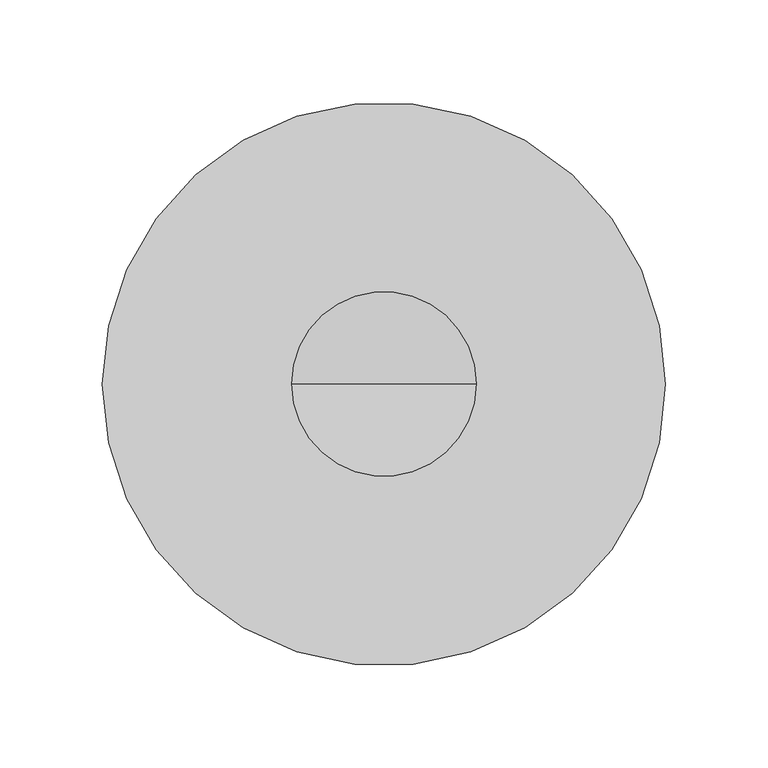
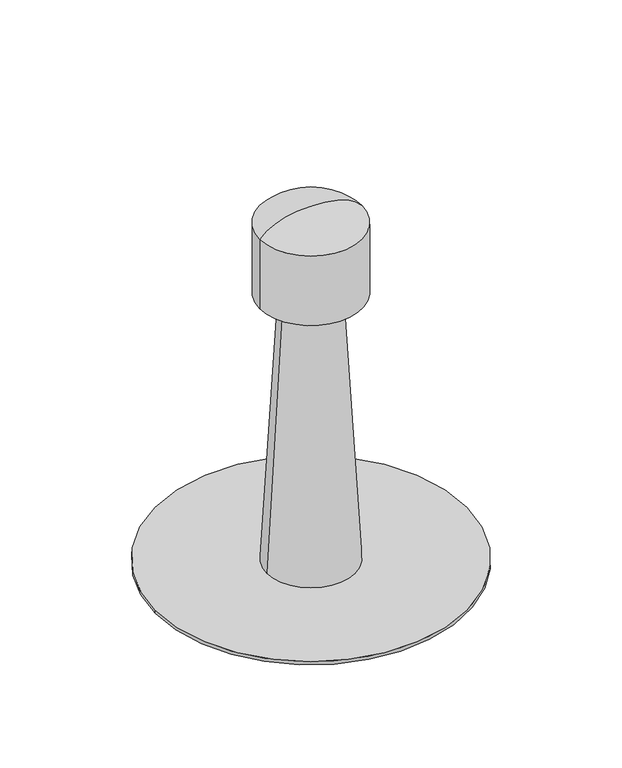
"""IFC4 building model written with IfcOpenShell, lengths in millimetres: proxy geometry, TN_ПВХ Кровельный аэратор : ПВХ аэратор кровельный 78х332 ТехноНИКОЛЬ."""

import ifcopenshell
import ifcopenshell.guid

model = None  # the IFC model being written
_history = None  # IfcOwnerHistory: only IFC2X3 demands one
_inside = {}  # id of a spatial element -> (the spatial element, [elements in it])
_under = {}  # id of a project, library or spatial element -> (it, [spatial elements below it])
_declared = {}  # id of a project -> (the project, [libraries it declares])
_typed = {}  # id of a type object -> (the type object, [elements of that type])
_made_of = {}  # id of a material, layer set ... -> (it, [elements and type objects made of it])


def new_model(schema):
    """Start an empty IFC model of exactly this schema.

    Asked for "IFC4X3", IfcOpenShell would pick the latest addendum, in which some entities
    have other attributes; the version numbers below select the first issue.
    IFC2X3 requires an IfcOwnerHistory on every rooted entity: one is made here for all.
    """
    global model, _history
    if schema == "IFC4X3":
        model = ifcopenshell.file(schema_version=(4, 3, 0, 0))
    else:
        model = ifcopenshell.file(schema=schema)
    _inside.clear()
    _under.clear()
    _declared.clear()
    _typed.clear()
    _made_of.clear()
    _history = None
    if model.schema == "IFC2X3":
        org = make("IfcOrganization", Name="unknown")
        user = make(
            "IfcPersonAndOrganization",
            ThePerson=make("IfcPerson", FamilyName="unknown"),
            TheOrganization=org,
        )
        app = make(
            "IfcApplication",
            ApplicationDeveloper=org,
            Version="unknown",
            ApplicationFullName="unknown",
            ApplicationIdentifier="unknown",
        )
        _history = make(
            "IfcOwnerHistory",
            OwningUser=user,
            OwningApplication=app,
            ChangeAction="ADDED",
            CreationDate=0,
        )
    return model


def make(cls, **values):
    """One entity of the class cls with the attributes given. An attribute that is None is left unset."""
    return model.create_entity(
        cls, **{name: value for name, value in values.items() if value is not None}
    )


def rooted(cls, **values):
    """An entity with a GlobalId (a new one), such as an element, a storey or a relation."""
    return make(cls, GlobalId=ifcopenshell.guid.new(), OwnerHistory=_history, **values)


def si_unit(unit_type, name, prefix=None):
    """IfcSIUnit, for example si_unit("LENGTHUNIT", "METRE", prefix="MILLI")."""
    return make("IfcSIUnit", UnitType=unit_type, Prefix=prefix, Name=name)


def assignment(units):
    """IfcUnitAssignment: the units of a project."""
    return None if units is None else make("IfcUnitAssignment", Units=units)


def point(xyz):
    """IfcCartesianPoint."""
    return None if xyz is None else make("IfcCartesianPoint", Coordinates=xyz)


def direction(xyz):
    """IfcDirection."""
    return None if xyz is None else make("IfcDirection", DirectionRatios=xyz)


def frame(location, z_axis=None, x_axis=None):
    """IfcAxis2Placement3D, a coordinate frame: its origin and axes. An axis left out is left unset."""
    return make(
        "IfcAxis2Placement3D",
        Location=point(location),
        Axis=direction(z_axis),
        RefDirection=direction(x_axis),
    )


def frame_2d(location, x_axis=None):
    """IfcAxis2Placement2D, a coordinate frame in the plane: its origin and x axis."""
    return make(
        "IfcAxis2Placement2D", Location=point(location), RefDirection=direction(x_axis)
    )


def origin():
    """The frame at (0, 0, 0) with its axes left unset."""
    return frame((0.0, 0.0, 0.0))


def origin_with_axes():
    """The frame at (0, 0, 0) with the z axis (0, 0, 1) and the x axis (1, 0, 0) written out."""
    return frame((0.0, 0.0, 0.0), z_axis=(0.0, 0.0, 1.0), x_axis=(1.0, 0.0, 0.0))


def origin_2d():
    """The frame at (0, 0) in the plane with its x axis left unset."""
    return frame_2d((0.0, 0.0))


def place(relative_to, where):
    """IfcLocalPlacement: puts the frame where relative to a parent placement (None: the world)."""
    return make(
        "IfcLocalPlacement", PlacementRelTo=relative_to, RelativePlacement=where
    )


def context(
    kind, dimensions, precision=None, world=None, true_north=None, identifier=None
):
    """IfcGeometricRepresentationContext, for example the 3D "Model" context."""
    return make(
        "IfcGeometricRepresentationContext",
        ContextIdentifier=identifier,
        ContextType=kind,
        CoordinateSpaceDimension=dimensions,
        Precision=precision,
        WorldCoordinateSystem=world,
        TrueNorth=true_north,
    )


def project(units=None, contexts=None):
    """IfcProject with its units and contexts."""
    return rooted(
        "IfcProject",
        Name="project",
        RepresentationContexts=contexts,
        UnitsInContext=assignment(units),
    )


def spatial(cls, under=None, at=None, **own):
    """A site, building, storey or space (cls), placed at a placement, below another one or the project."""
    s = rooted(cls, ObjectPlacement=at, **own)
    if under is not None:
        _under.setdefault(under.id(), (under, []))[1].append(s)
    return s


def polyline(points):
    """IfcPolyline through the points."""
    return make("IfcPolyline", Points=[point(p) for p in points])


def circle_curve(where, radius):
    """IfcCircle in the frame where."""
    return make("IfcCircle", Position=where, Radius=radius)


def trimmed(basis, trim1, trim2, sense, master):
    """IfcTrimmedCurve: the piece of a basis curve between two trims."""
    return make(
        "IfcTrimmedCurve",
        BasisCurve=basis,
        Trim1=trim1,
        Trim2=trim2,
        SenseAgreement=sense,
        MasterRepresentation=master,
    )


def segment(curve, same_sense, transition):
    """IfcCompositeCurveSegment."""
    return make(
        "IfcCompositeCurveSegment",
        Transition=transition,
        SameSense=same_sense,
        ParentCurve=curve,
    )


def composite_curve(segments, self_intersect=None):
    """IfcCompositeCurve: segments joined end to end."""
    return make("IfcCompositeCurve", Segments=segments, SelfIntersect=self_intersect)


def outline(outer, holes=None, kind="AREA"):
    """IfcArbitraryClosedProfileDef: a profile drawn as a closed curve; with holes, ...WithVoids."""
    if holes is None:
        return make("IfcArbitraryClosedProfileDef", ProfileType=kind, OuterCurve=outer)
    return make(
        "IfcArbitraryProfileDefWithVoids",
        ProfileType=kind,
        OuterCurve=outer,
        InnerCurves=holes,
    )


def extrude(swept, where, along, depth):
    """IfcExtrudedAreaSolid: the profile swept, set in the frame where, extruded along a direction by depth."""
    return make(
        "IfcExtrudedAreaSolid",
        SweptArea=swept,
        Position=where,
        ExtrudedDirection=direction(along),
        Depth=depth,
    )


def shape(context_of_items, identifier, shape_type, items):
    """IfcShapeRepresentation: the items that make up one representation, for example the "Body"."""
    return make(
        "IfcShapeRepresentation",
        ContextOfItems=context_of_items,
        RepresentationIdentifier=identifier,
        RepresentationType=shape_type,
        Items=items,
    )


def source(mapping_origin, context_of_items, identifier, shape_type, items):
    """IfcRepresentationMap: a shape defined once, which mapped items show again and again."""
    return make(
        "IfcRepresentationMap",
        MappingOrigin=mapping_origin,
        MappedRepresentation=shape(context_of_items, identifier, shape_type, items),
    )


def transform(
    local_origin,
    x_axis=None,
    y_axis=None,
    z_axis=None,
    scale=None,
    scale2=None,
    scale3=None,
    uniform=True,
):
    """IfcCartesianTransformationOperator3D, or its non-uniform kind. x_axis, y_axis, z_axis: its Axis1, 2, 3."""
    if uniform:
        return make(
            "IfcCartesianTransformationOperator3D",
            Axis1=direction(x_axis),
            Axis2=direction(y_axis),
            LocalOrigin=point(local_origin),
            Scale=scale,
            Axis3=direction(z_axis),
        )
    return make(
        "IfcCartesianTransformationOperator3DnonUniform",
        Axis1=direction(x_axis),
        Axis2=direction(y_axis),
        LocalOrigin=point(local_origin),
        Scale=scale,
        Axis3=direction(z_axis),
        Scale2=scale2,
        Scale3=scale3,
    )


def mapped(mapping_source, mapping_target):
    """IfcMappedItem: shows the shape of a source again, moved by a transform."""
    return make(
        "IfcMappedItem", MappingSource=mapping_source, MappingTarget=mapping_target
    )


def made_of(thing, what):
    """Note that an element or type object is made of a material, layer set ...; save() writes the relation."""
    if what is not None:
        _made_of.setdefault(what.id(), (what, []))[1].append(thing)
    return thing


def element(
    cls,
    number,
    at=None,
    inside=None,
    cuts=None,
    type_object=None,
    material=None,
    context=None,
    identifier="Body",
    shape_type=None,
    held_by="IfcProductDefinitionShape",
    body=None,
    shapes=None,
    **own,
):
    """One element of the class cls, such as IfcWall. Its Tag is "e" and its number.

    at: its placement. inside: the storey or other place that contains it. cuts: it is an
    opening in that element (IfcRelVoidsElement). A single representation is given by context,
    identifier, shape_type and body (its items); several are given by shapes. held_by: the class
    of the entity that holds the representations. save() writes the other relations.
    """
    e = rooted(cls, Tag="e%d" % number, ObjectPlacement=at, **own)
    if body is not None:
        shapes = [shape(context, identifier, shape_type, body)]
    if shapes is not None:
        e.Representation = make(held_by, Representations=shapes)
    if inside is not None:
        _inside.setdefault(inside.id(), (inside, []))[1].append(e)
    if cuts is not None:
        rooted(
            "IfcRelVoidsElement", RelatingBuildingElement=cuts, RelatedOpeningElement=e
        )
    if type_object is not None:
        _typed.setdefault(type_object.id(), (type_object, []))[1].append(e)
    return made_of(e, material)


def aggregate(whole, parts):
    """IfcRelAggregates: a whole, such as a stair, and the parts it consists of."""
    return rooted("IfcRelAggregates", RelatingObject=whole, RelatedObjects=parts)


def save(model, path):
    """Write the relations noted so far, then the file.

    IfcRelAggregates (storeys below a building ...), IfcRelContainedInSpatialStructure (elements
    in a storey), IfcRelDefinesByType, IfcRelAssociatesMaterial and IfcRelDeclares: one each for
    every whole, place, type object, material and project.
    """
    for whole, parts in _under.values():
        aggregate(whole, parts)
    for where, things in _inside.values():
        rooted(
            "IfcRelContainedInSpatialStructure",
            RelatedElements=things,
            RelatingStructure=where,
        )
    for kind, things in _typed.values():
        rooted("IfcRelDefinesByType", RelatedObjects=things, RelatingType=kind)
    for what, things in _made_of.values():
        rooted("IfcRelAssociatesMaterial", RelatedObjects=things, RelatingMaterial=what)
    for by, libraries in _declared.values():
        rooted("IfcRelDeclares", RelatingContext=by, RelatedDefinitions=libraries)
    model.write(path)


def plane_surface(at):
    """IfcPlane: the flat surface through the origin of the frame at, square to its z axis."""
    return make("IfcPlane", Position=at)


def cylinder_surface(at, radius):
    """IfcCylindricalSurface: all points at the distance radius from the z axis of the frame at."""
    return make("IfcCylindricalSurface", Position=at, Radius=radius)


def revolved_surface(curve, axis_point, axis_direction):
    """IfcSurfaceOfRevolution: the curve turned about the line through axis_point along axis_direction."""
    return make(
        "IfcSurfaceOfRevolution",
        SweptCurve=make("IfcArbitraryOpenProfileDef", ProfileType="CURVE", Curve=curve),
        AxisPosition=make("IfcAxis1Placement", Location=point(axis_point), Axis=direction(axis_direction)),
    )


def spline_curve(degree, points, multiplicities, knots, weights=None):
    """IfcBSplineCurveWithKnots; with weights, IfcRationalBSplineCurveWithKnots."""
    own = dict(
        Degree=degree,
        ControlPointsList=[point(p) for p in points],
        CurveForm="UNSPECIFIED",
        ClosedCurve=False,
        SelfIntersect=False,
        KnotMultiplicities=multiplicities,
        Knots=knots,
        KnotSpec="UNSPECIFIED",
    )
    if weights is None:
        return make("IfcBSplineCurveWithKnots", **own)
    return make("IfcRationalBSplineCurveWithKnots", WeightsData=weights, **own)


def advanced_brep(points, edges, surfaces, faces):
    """IfcAdvancedBrep: a solid bounded by faces that lie on surfaces and meet in shared edges.

    An edge is (start, end): straight between two places in points (the first is 0);
    or (start, end, curve); or (start, end, curve, False) where it runs against its curve.
    A face is (place in surfaces, loops), or (place, loops, False) where it looks against
    its surface's normal. A loop lists edges by number (the first is 1), with a minus sign
    where the edge is run from its end to its start. The first loop is the outer one.
    """
    corners = [point(p) for p in points]
    vertices = [make("IfcVertexPoint", VertexGeometry=c) for c in corners]
    made = []
    for start, end, *more in edges:
        made.append(
            make(
                "IfcEdgeCurve",
                EdgeStart=vertices[start],
                EdgeEnd=vertices[end],
                EdgeGeometry=more[0] if more else make("IfcPolyline", Points=[corners[start], corners[end]]),
                SameSense=more[1] if len(more) > 1 else True,
            )
        )
    hull = []
    for where, loops, *sense in faces:
        bounds = []
        for j, loop in enumerate(loops):
            ring = [make("IfcOrientedEdge", EdgeElement=made[abs(k) - 1], Orientation=k > 0) for k in loop]
            bounds.append(
                make(
                    "IfcFaceOuterBound" if j == 0 else "IfcFaceBound",
                    Bound=make("IfcEdgeLoop", EdgeList=ring),
                    Orientation=True,
                )
            )
        hull.append(make("IfcAdvancedFace", Bounds=bounds, FaceSurface=surfaces[where], SameSense=sense[0] if sense else True))
    return make("IfcAdvancedBrep", Outer=make("IfcClosedShell", CfsFaces=hull))


def specialty_equipment_692bb2d6(model_context):
    return source(origin(), model_context, "Body", "SolidModel", [
        advanced_brep(
        [(25.0, 0.0, 252.0), (-25.0, 0.0, 252.0), (0.0, 0.0, 252.0), (0.0, 0.0, 3.0), (-39.0, 0.0, 3.0), (39.0, 0.0, 3.0)],
        [
            (0, 1, circle_curve(frame((0.0, 0.0, 252.0), z_axis=(0.0, 0.0, 1.0), x_axis=(-1.0, 0.0, 0.0)), 25.0)),
            (1, 2),
            (2, 0),
            (1, 0, circle_curve(frame((0.0, 0.0, 252.0), z_axis=(0.0, 0.0, 1.0), x_axis=(-1.0, 0.0, 0.0)), 25.0)),
            (3, 4),
            (4, 5, circle_curve(frame((0.0, 0.0, 3.0), z_axis=(0.0, 0.0, -1.0), x_axis=(-1.0, 0.0, 0.0)), 39.0)),
            (5, 3),
            (5, 4, circle_curve(frame((0.0, 0.0, 3.0), z_axis=(0.0, 0.0, -1.0), x_axis=(-1.0, 0.0, 0.0)), 39.0)),
            (4, 1),
            (0, 5),
        ],
        [
            plane_surface(frame((0.0, 0.0, 252.0), z_axis=(0.0, 0.0, 1.0), x_axis=(-1.0, 0.0, 0.0))),
            plane_surface(frame((0.0, 0.0, 3.0), z_axis=(0.0, 0.0, -1.0), x_axis=(-1.0, 0.0, 0.0))),
            revolved_surface(polyline([(-25.0, 0.0, 252.0), (-39.0, 0.0, 3.0)]), (0.0, 0.0, -2.0), (0.0, 0.0, -1.0)),
        ],
        [
            (0, [[1, 2, 3]]),
            (0, [[4, -3, -2]]),
            (1, [[5, 6, 7]]),
            (1, [[-7, 8, -5]]),
            (2, [[-6, 9, -1, 10]]),
            (2, [[-8, -10, -4, -9]]),
        ],
    ),
        advanced_brep(
        [(0.0, 0.0, 252.0), (-45.0, 0.0, 252.0), (45.0, 0.0, 252.0), (45.0, 0.0, 317.0), (-45.0, 0.0, 317.0), (0.0, 0.0, 332.0)],
        [
            (0, 1),
            (1, 2, circle_curve(frame((0.0, 0.0, 252.0), z_axis=(0.0, 0.0, -1.0), x_axis=(-1.0, 0.0, 0.0)), 45.0)),
            (2, 0),
            (2, 1, circle_curve(frame((0.0, 0.0, 252.0), z_axis=(0.0, 0.0, -1.0), x_axis=(-1.0, 0.0, 0.0)), 45.0)),
            (3, 4, circle_curve(frame((0.0, 0.0, 317.0), z_axis=(0.0, 0.0, 1.0), x_axis=(-1.0, 0.0, 0.0)), 45.0)),
            (4, 5, spline_curve(3, [(-45.0, 0.0, 317.0), (-36.982596383, 0.0, 326.999999999), (-21.982596382, 0.0, 332.0), (0.0, 0.0, 332.0)], [4, 4], [0.0, 0.08562924216502088])),
            (5, 3, spline_curve(3, [(0.0, 0.0, 332.0), (21.982596382, 0.0, 332.0), (36.982596383, 0.0, 326.999999999), (45.0, 0.0, 317.0)], [4, 4], [0.0, 0.08562924216502088])),
            (4, 3, circle_curve(frame((0.0, 0.0, 317.0), z_axis=(0.0, 0.0, 1.0), x_axis=(-1.0, 0.0, 0.0)), 45.0)),
            (1, 4),
            (3, 2),
        ],
        [
            plane_surface(frame((0.0, 0.0, 252.0), z_axis=(0.0, 0.0, -1.0), x_axis=(-1.0, 0.0, 0.0))),
            revolved_surface(spline_curve(3, [(0.0, 0.0, 332.0), (-21.982596382, 0.0, 332.0), (-36.982596383, 0.0, 326.999999999), (-45.0, 0.0, 317.0)], [4, 4], [0.0, 0.08562924216502088]), (0.0, 0.0, 347.0), (0.0, 0.0, -1.0)),
            cylinder_surface(frame((0.0, 0.0, 347.0), z_axis=(0.0, 0.0, -1.0), x_axis=(-1.0, 0.0, 0.0)), 45.0),
        ],
        [
            (0, [[1, 2, 3]]),
            (0, [[-3, 4, -1]]),
            (1, [[5, 6, 7]]),
            (1, [[8, -7, -6]]),
            (2, [[-2, 9, -5, 10]]),
            (2, [[-4, -10, -8, -9]]),
        ],
    ),
        extrude(outline(composite_curve([segment(trimmed(circle_curve(origin_2d(), 137.5), [point((-137.5, 0.0))], [point((137.5, 0.0))], False, "CARTESIAN"), True, "CONTINUOUS"), segment(trimmed(circle_curve(origin_2d(), 137.5), [point((137.5, 0.0))], [point((-137.5, 0.0))], False, "CARTESIAN"), True, "CONTINUOUS")], self_intersect=False)), origin_with_axes(), (0.0, 0.0, 1.0), 3.0),
    ])


if __name__ == "__main__":
    model = new_model("IFC4")
    model_context = context("Model", 3, world=origin())
    ifc_project = project(units=[si_unit("LENGTHUNIT", "METRE", prefix="MILLI")], contexts=[model_context])
    site = spatial("IfcSite", under=ifc_project)
    building = spatial("IfcBuilding", under=site)
    placement = place(None, origin())
    specialty_equipment_shape = specialty_equipment_692bb2d6(model_context)
    element("IfcBuildingElementProxy", 1, Name="TN_ПВХ Кровельный аэратор : ПВХ аэратор кровельный 78х332 ТехноНИКОЛЬ", ObjectType="TN_ПВХ Кровельный аэратор : ПВХ аэратор кровельный 78х332 ТехноНИКОЛЬ", at=placement, inside=building, context=model_context, shape_type="MappedRepresentation", body=[
        mapped(specialty_equipment_shape, transform((0.0, 0.0, 0.0), x_axis=(1.0, 0.0, 0.0), y_axis=(0.0, 1.0, 0.0), z_axis=(0.0, 0.0, 1.0))),
    ])
    save(model, "model.ifc")

# Revit data of these elements
# Type "TN_ПВХ Кровельный аэратор : ПВХ аэратор кровельный 78х332 ТехноНИКОЛЬ"
#   ADSK_Группирование = "Комплектующие и воронки"
#   Description = "ПВХ аэратор применяется при устройстве либо санации «дышащих» плоских кровель. Предназначены для отвода водяных паров, проникающих под гидроизоляционный слой кровли. Предотвращают образование вздутий и последующего разрыва защитного кровельного материала, тем самым увеличивая срок службы гидроизоляционного ковра.  Данный Аэратор симеет жесткий  корпус; колпак на аэраторе имеет жёсткое фиксирование, что исключит его срыв ветром; высота аэратора позволяет в весенний период при таянии сугробов исключит попадание воды через отводящую трубу аэратора.  Устанавливаются аэраторы данного типа из расчета не менее 1 шт. на 235 м² кровли. Расстояние между аэраторами не должно превышать 12 метров."
#   Manufacturer = "ТехноНИКОЛЬ"
#   ADSK_Обозначение = "ТехноНИКОЛЬ"
#   ADSK_Наименование = "ПВХ аэратор кровельный 78х332мм"
#   ADSK_Код изделия = "046223"
#   ADSK_Завод-изготовитель = "ТехноНИКОЛЬ"
#   ADSK_Единица измерения = "шт."
#   ADSK_Группирование = "Комплектующие и воронки"
#   ADSK_URL страницы изделия = ""
#   ADSK_URL документации изделия = ""
#   Default Elevation = 1219.2 mm
#   ADSK_Размер_Ширина = 39 mm
#   ADSK_Размер_Высота = 332 mm
#   ADSK_Масса = 0.83
#   ADSK_Количество = 1
#   Материал = TN_ПВХ_ТемноСерый
#   URL = ""
# Element 1 (IfcBuildingElementProxy, "TN_ПВХ Кровельный аэратор : ПВХ аэратор кровельный 78х332 ТехноНИКОЛЬ")
#   Materials on its faces: "TN_ПВХ_ТемноСерый"
# Materials
#   "TN_ПВХ_ТемноСерый": class "Типовые", colour RGB 100 100 100, transparency 0, Cost = 0
